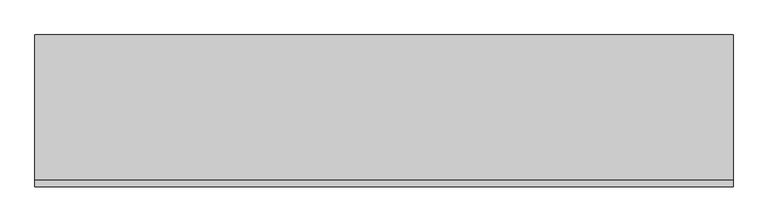
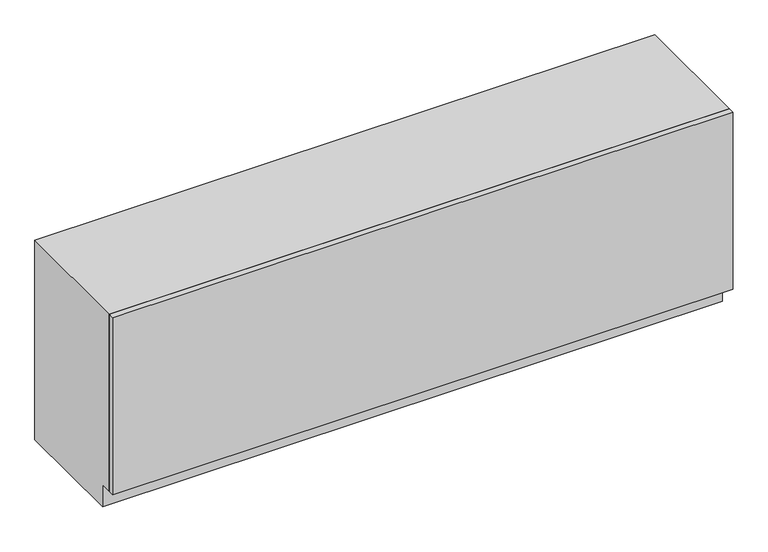
"""IFC4 building model written with IfcOpenShell, lengths in millimetres: furniture geometry, OD_CW_Base Cabinet : OD_CW_Base Cabinet."""

import ifcopenshell
import ifcopenshell.guid

model = None  # the IFC model being written
_history = None  # IfcOwnerHistory: only IFC2X3 demands one
_inside = {}  # id of a spatial element -> (the spatial element, [elements in it])
_under = {}  # id of a project, library or spatial element -> (it, [spatial elements below it])
_declared = {}  # id of a project -> (the project, [libraries it declares])
_typed = {}  # id of a type object -> (the type object, [elements of that type])
_made_of = {}  # id of a material, layer set ... -> (it, [elements and type objects made of it])


def new_model(schema):
    """Start an empty IFC model of exactly this schema.

    Asked for "IFC4X3", IfcOpenShell would pick the latest addendum, in which some entities
    have other attributes; the version numbers below select the first issue.
    IFC2X3 requires an IfcOwnerHistory on every rooted entity: one is made here for all.
    """
    global model, _history
    if schema == "IFC4X3":
        model = ifcopenshell.file(schema_version=(4, 3, 0, 0))
    else:
        model = ifcopenshell.file(schema=schema)
    _inside.clear()
    _under.clear()
    _declared.clear()
    _typed.clear()
    _made_of.clear()
    _history = None
    if model.schema == "IFC2X3":
        org = make("IfcOrganization", Name="unknown")
        user = make(
            "IfcPersonAndOrganization",
            ThePerson=make("IfcPerson", FamilyName="unknown"),
            TheOrganization=org,
        )
        app = make(
            "IfcApplication",
            ApplicationDeveloper=org,
            Version="unknown",
            ApplicationFullName="unknown",
            ApplicationIdentifier="unknown",
        )
        _history = make(
            "IfcOwnerHistory",
            OwningUser=user,
            OwningApplication=app,
            ChangeAction="ADDED",
            CreationDate=0,
        )
    return model


def make(cls, **values):
    """One entity of the class cls with the attributes given. An attribute that is None is left unset."""
    return model.create_entity(
        cls, **{name: value for name, value in values.items() if value is not None}
    )


def rooted(cls, **values):
    """An entity with a GlobalId (a new one), such as an element, a storey or a relation."""
    return make(cls, GlobalId=ifcopenshell.guid.new(), OwnerHistory=_history, **values)


def si_unit(unit_type, name, prefix=None):
    """IfcSIUnit, for example si_unit("LENGTHUNIT", "METRE", prefix="MILLI")."""
    return make("IfcSIUnit", UnitType=unit_type, Prefix=prefix, Name=name)


def assignment(units):
    """IfcUnitAssignment: the units of a project."""
    return None if units is None else make("IfcUnitAssignment", Units=units)


def point(xyz):
    """IfcCartesianPoint."""
    return None if xyz is None else make("IfcCartesianPoint", Coordinates=xyz)


def direction(xyz):
    """IfcDirection."""
    return None if xyz is None else make("IfcDirection", DirectionRatios=xyz)


def frame(location, z_axis=None, x_axis=None):
    """IfcAxis2Placement3D, a coordinate frame: its origin and axes. An axis left out is left unset."""
    return make(
        "IfcAxis2Placement3D",
        Location=point(location),
        Axis=direction(z_axis),
        RefDirection=direction(x_axis),
    )


def origin():
    """The frame at (0, 0, 0) with its axes left unset."""
    return frame((0.0, 0.0, 0.0))


def place(relative_to, where):
    """IfcLocalPlacement: puts the frame where relative to a parent placement (None: the world)."""
    return make(
        "IfcLocalPlacement", PlacementRelTo=relative_to, RelativePlacement=where
    )


def context(
    kind, dimensions, precision=None, world=None, true_north=None, identifier=None
):
    """IfcGeometricRepresentationContext, for example the 3D "Model" context."""
    return make(
        "IfcGeometricRepresentationContext",
        ContextIdentifier=identifier,
        ContextType=kind,
        CoordinateSpaceDimension=dimensions,
        Precision=precision,
        WorldCoordinateSystem=world,
        TrueNorth=true_north,
    )


def project(units=None, contexts=None):
    """IfcProject with its units and contexts."""
    return rooted(
        "IfcProject",
        Name="project",
        RepresentationContexts=contexts,
        UnitsInContext=assignment(units),
    )


def spatial(cls, under=None, at=None, **own):
    """A site, building, storey or space (cls), placed at a placement, below another one or the project."""
    s = rooted(cls, ObjectPlacement=at, **own)
    if under is not None:
        _under.setdefault(under.id(), (under, []))[1].append(s)
    return s


def polyline(points):
    """IfcPolyline through the points."""
    return make("IfcPolyline", Points=[point(p) for p in points])


def outline(outer, holes=None, kind="AREA"):
    """IfcArbitraryClosedProfileDef: a profile drawn as a closed curve; with holes, ...WithVoids."""
    if holes is None:
        return make("IfcArbitraryClosedProfileDef", ProfileType=kind, OuterCurve=outer)
    return make(
        "IfcArbitraryProfileDefWithVoids",
        ProfileType=kind,
        OuterCurve=outer,
        InnerCurves=holes,
    )


def extrude(swept, where, along, depth):
    """IfcExtrudedAreaSolid: the profile swept, set in the frame where, extruded along a direction by depth."""
    return make(
        "IfcExtrudedAreaSolid",
        SweptArea=swept,
        Position=where,
        ExtrudedDirection=direction(along),
        Depth=depth,
    )


def shape(context_of_items, identifier, shape_type, items):
    """IfcShapeRepresentation: the items that make up one representation, for example the "Body"."""
    return make(
        "IfcShapeRepresentation",
        ContextOfItems=context_of_items,
        RepresentationIdentifier=identifier,
        RepresentationType=shape_type,
        Items=items,
    )


def source(mapping_origin, context_of_items, identifier, shape_type, items):
    """IfcRepresentationMap: a shape defined once, which mapped items show again and again."""
    return make(
        "IfcRepresentationMap",
        MappingOrigin=mapping_origin,
        MappedRepresentation=shape(context_of_items, identifier, shape_type, items),
    )


def transform(
    local_origin,
    x_axis=None,
    y_axis=None,
    z_axis=None,
    scale=None,
    scale2=None,
    scale3=None,
    uniform=True,
):
    """IfcCartesianTransformationOperator3D, or its non-uniform kind. x_axis, y_axis, z_axis: its Axis1, 2, 3."""
    if uniform:
        return make(
            "IfcCartesianTransformationOperator3D",
            Axis1=direction(x_axis),
            Axis2=direction(y_axis),
            LocalOrigin=point(local_origin),
            Scale=scale,
            Axis3=direction(z_axis),
        )
    return make(
        "IfcCartesianTransformationOperator3DnonUniform",
        Axis1=direction(x_axis),
        Axis2=direction(y_axis),
        LocalOrigin=point(local_origin),
        Scale=scale,
        Axis3=direction(z_axis),
        Scale2=scale2,
        Scale3=scale3,
    )


def mapped(mapping_source, mapping_target):
    """IfcMappedItem: shows the shape of a source again, moved by a transform."""
    return make(
        "IfcMappedItem", MappingSource=mapping_source, MappingTarget=mapping_target
    )


def made_of(thing, what):
    """Note that an element or type object is made of a material, layer set ...; save() writes the relation."""
    if what is not None:
        _made_of.setdefault(what.id(), (what, []))[1].append(thing)
    return thing


def element(
    cls,
    number,
    at=None,
    inside=None,
    cuts=None,
    type_object=None,
    material=None,
    context=None,
    identifier="Body",
    shape_type=None,
    held_by="IfcProductDefinitionShape",
    body=None,
    shapes=None,
    **own,
):
    """One element of the class cls, such as IfcWall. Its Tag is "e" and its number.

    at: its placement. inside: the storey or other place that contains it. cuts: it is an
    opening in that element (IfcRelVoidsElement). A single representation is given by context,
    identifier, shape_type and body (its items); several are given by shapes. held_by: the class
    of the entity that holds the representations. save() writes the other relations.
    """
    e = rooted(cls, Tag="e%d" % number, ObjectPlacement=at, **own)
    if body is not None:
        shapes = [shape(context, identifier, shape_type, body)]
    if shapes is not None:
        e.Representation = make(held_by, Representations=shapes)
    if inside is not None:
        _inside.setdefault(inside.id(), (inside, []))[1].append(e)
    if cuts is not None:
        rooted(
            "IfcRelVoidsElement", RelatingBuildingElement=cuts, RelatedOpeningElement=e
        )
    if type_object is not None:
        _typed.setdefault(type_object.id(), (type_object, []))[1].append(e)
    return made_of(e, material)


def aggregate(whole, parts):
    """IfcRelAggregates: a whole, such as a stair, and the parts it consists of."""
    return rooted("IfcRelAggregates", RelatingObject=whole, RelatedObjects=parts)


def save(model, path):
    """Write the relations noted so far, then the file.

    IfcRelAggregates (storeys below a building ...), IfcRelContainedInSpatialStructure (elements
    in a storey), IfcRelDefinesByType, IfcRelAssociatesMaterial and IfcRelDeclares: one each for
    every whole, place, type object, material and project.
    """
    for whole, parts in _under.values():
        aggregate(whole, parts)
    for where, things in _inside.values():
        rooted(
            "IfcRelContainedInSpatialStructure",
            RelatedElements=things,
            RelatingStructure=where,
        )
    for kind, things in _typed.values():
        rooted("IfcRelDefinesByType", RelatedObjects=things, RelatingType=kind)
    for what, things in _made_of.values():
        rooted("IfcRelAssociatesMaterial", RelatedObjects=things, RelatingMaterial=what)
    for by, libraries in _declared.values():
        rooted("IfcRelDeclares", RelatingContext=by, RelatedDefinitions=libraries)
    model.write(path)


def furniture_05bdc3bb(model_context):
    return source(origin(), model_context, "Body", "SweptSolid", [
        extrude(outline(polyline([(18.7377049, 49.9884781), (2710.6718262, 49.9884781), (2710.6718262, 24.5884781), (18.7377049, 24.5884781), (18.7377049, 49.9884781)])), frame((0.0, 0.0, 101.6), z_axis=(0.0, 0.0, 1.0), x_axis=(1.0, 0.0, 0.0)), (0.0, 0.0, 1.0), 812.8),
        extrude(outline(polyline([(49.9884781, 914.4), (609.6, 914.4), (609.6, 0.0), (100.7884781, 0.0), (100.7884781, 101.6), (49.9884781, 101.6), (49.9884781, 914.4)])), frame((18.7377049, 0.0, 0.0), z_axis=(1.0, 0.0, 0.0), x_axis=(0.0, 1.0, 0.0)), (0.0, 0.0, 1.0), 2691.9341213),
    ])


if __name__ == "__main__":
    model = new_model("IFC4")
    model_context = context("Model", 3, world=origin())
    ifc_project = project(units=[si_unit("LENGTHUNIT", "METRE", prefix="MILLI")], contexts=[model_context])
    site = spatial("IfcSite", under=ifc_project)
    building = spatial("IfcBuilding", under=site)
    placement = place(None, origin())
    furniture_shape = furniture_05bdc3bb(model_context)
    element("IfcFurniture", 1, ObjectType="OD_CW_Base Cabinet : OD_CW_Base Cabinet", at=placement, inside=building, context=model_context, shape_type="MappedRepresentation", body=[
        mapped(furniture_shape, transform((0.0, 0.0, 0.0), x_axis=(1.0, 0.0, 0.0), y_axis=(0.0, 1.0, 0.0), z_axis=(0.0, 0.0, 1.0))),
    ])
    save(model, "model.ifc")

# Revit data of these elements
# Type "OD_CW_Base Cabinet : OD_CW_Base Cabinet"
#   OD_CW_Width [instance default] = 2' - 10"
#   OD_CW_Length [instance default] = 8' - 0"
#   OD_CW_Height [instance default] = 2' - 3"
#   Depth = 2' - 0"
#   Height = 3' - 0"
#   Width = 4' - 0"
#   OD_CW_Material_Front Panel [instance default] = none
#   OD_CW_Material_Body [instance default] = none
# Element 1 (IfcFurniture, "OD_CW_Base Cabinet : OD_CW_Base Cabinet")
#   OD_CW_Width = 1' - 11.03195"
#   OD_CW_Length = 8' - 9.98166"
#   OD_CW_Height = 3' - 0"
#   OD_CW_Material_Body = WINE STATION
#   Materials on its faces: "WINE STATION", "CASEWORK"
# Materials
#   "WINE STATION": class "Generic", colour RGB 187 187 187, transparency 0, Cost = 0
#   "CASEWORK": class "Generic", colour RGB 181 181 181, transparency 0, Cost = 0
